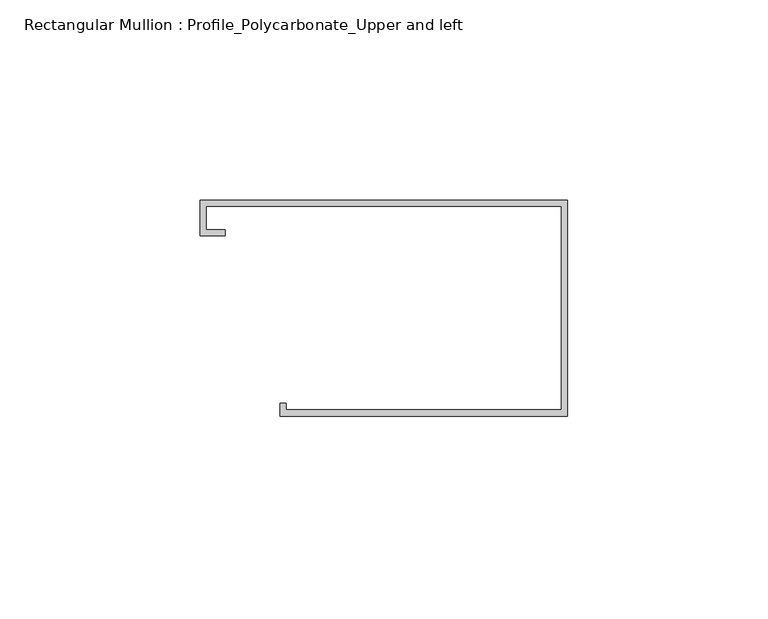
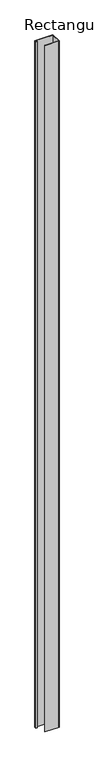
"""IFC4 building model written with IfcOpenShell, lengths in millimetres: member geometry, Rectangular Mullion : Profile_Polycarbonate_Upper and left."""

import ifcopenshell
import ifcopenshell.guid

model = None  # the IFC model being written
_history = None  # IfcOwnerHistory: only IFC2X3 demands one
_inside = {}  # id of a spatial element -> (the spatial element, [elements in it])
_under = {}  # id of a project, library or spatial element -> (it, [spatial elements below it])
_declared = {}  # id of a project -> (the project, [libraries it declares])
_typed = {}  # id of a type object -> (the type object, [elements of that type])
_made_of = {}  # id of a material, layer set ... -> (it, [elements and type objects made of it])


def new_model(schema):
    """Start an empty IFC model of exactly this schema.

    Asked for "IFC4X3", IfcOpenShell would pick the latest addendum, in which some entities
    have other attributes; the version numbers below select the first issue.
    IFC2X3 requires an IfcOwnerHistory on every rooted entity: one is made here for all.
    """
    global model, _history
    if schema == "IFC4X3":
        model = ifcopenshell.file(schema_version=(4, 3, 0, 0))
    else:
        model = ifcopenshell.file(schema=schema)
    _inside.clear()
    _under.clear()
    _declared.clear()
    _typed.clear()
    _made_of.clear()
    _history = None
    if model.schema == "IFC2X3":
        org = make("IfcOrganization", Name="unknown")
        user = make(
            "IfcPersonAndOrganization",
            ThePerson=make("IfcPerson", FamilyName="unknown"),
            TheOrganization=org,
        )
        app = make(
            "IfcApplication",
            ApplicationDeveloper=org,
            Version="unknown",
            ApplicationFullName="unknown",
            ApplicationIdentifier="unknown",
        )
        _history = make(
            "IfcOwnerHistory",
            OwningUser=user,
            OwningApplication=app,
            ChangeAction="ADDED",
            CreationDate=0,
        )
    return model


def make(cls, **values):
    """One entity of the class cls with the attributes given. An attribute that is None is left unset."""
    return model.create_entity(
        cls, **{name: value for name, value in values.items() if value is not None}
    )


def rooted(cls, **values):
    """An entity with a GlobalId (a new one), such as an element, a storey or a relation."""
    return make(cls, GlobalId=ifcopenshell.guid.new(), OwnerHistory=_history, **values)


def si_unit(unit_type, name, prefix=None):
    """IfcSIUnit, for example si_unit("LENGTHUNIT", "METRE", prefix="MILLI")."""
    return make("IfcSIUnit", UnitType=unit_type, Prefix=prefix, Name=name)


def assignment(units):
    """IfcUnitAssignment: the units of a project."""
    return None if units is None else make("IfcUnitAssignment", Units=units)


def point(xyz):
    """IfcCartesianPoint."""
    return None if xyz is None else make("IfcCartesianPoint", Coordinates=xyz)


def direction(xyz):
    """IfcDirection."""
    return None if xyz is None else make("IfcDirection", DirectionRatios=xyz)


def frame(location, z_axis=None, x_axis=None):
    """IfcAxis2Placement3D, a coordinate frame: its origin and axes. An axis left out is left unset."""
    return make(
        "IfcAxis2Placement3D",
        Location=point(location),
        Axis=direction(z_axis),
        RefDirection=direction(x_axis),
    )


def origin():
    """The frame at (0, 0, 0) with its axes left unset."""
    return frame((0.0, 0.0, 0.0))


def place(relative_to, where):
    """IfcLocalPlacement: puts the frame where relative to a parent placement (None: the world)."""
    return make(
        "IfcLocalPlacement", PlacementRelTo=relative_to, RelativePlacement=where
    )


def context(
    kind, dimensions, precision=None, world=None, true_north=None, identifier=None
):
    """IfcGeometricRepresentationContext, for example the 3D "Model" context."""
    return make(
        "IfcGeometricRepresentationContext",
        ContextIdentifier=identifier,
        ContextType=kind,
        CoordinateSpaceDimension=dimensions,
        Precision=precision,
        WorldCoordinateSystem=world,
        TrueNorth=true_north,
    )


def project(units=None, contexts=None):
    """IfcProject with its units and contexts."""
    return rooted(
        "IfcProject",
        Name="project",
        RepresentationContexts=contexts,
        UnitsInContext=assignment(units),
    )


def spatial(cls, under=None, at=None, **own):
    """A site, building, storey or space (cls), placed at a placement, below another one or the project."""
    s = rooted(cls, ObjectPlacement=at, **own)
    if under is not None:
        _under.setdefault(under.id(), (under, []))[1].append(s)
    return s


def polyline(points):
    """IfcPolyline through the points."""
    return make("IfcPolyline", Points=[point(p) for p in points])


def outline(outer, holes=None, kind="AREA"):
    """IfcArbitraryClosedProfileDef: a profile drawn as a closed curve; with holes, ...WithVoids."""
    if holes is None:
        return make("IfcArbitraryClosedProfileDef", ProfileType=kind, OuterCurve=outer)
    return make(
        "IfcArbitraryProfileDefWithVoids",
        ProfileType=kind,
        OuterCurve=outer,
        InnerCurves=holes,
    )


def extrude(swept, where, along, depth):
    """IfcExtrudedAreaSolid: the profile swept, set in the frame where, extruded along a direction by depth."""
    return make(
        "IfcExtrudedAreaSolid",
        SweptArea=swept,
        Position=where,
        ExtrudedDirection=direction(along),
        Depth=depth,
    )


def shape(context_of_items, identifier, shape_type, items):
    """IfcShapeRepresentation: the items that make up one representation, for example the "Body"."""
    return make(
        "IfcShapeRepresentation",
        ContextOfItems=context_of_items,
        RepresentationIdentifier=identifier,
        RepresentationType=shape_type,
        Items=items,
    )


def source(mapping_origin, context_of_items, identifier, shape_type, items):
    """IfcRepresentationMap: a shape defined once, which mapped items show again and again."""
    return make(
        "IfcRepresentationMap",
        MappingOrigin=mapping_origin,
        MappedRepresentation=shape(context_of_items, identifier, shape_type, items),
    )


def transform(
    local_origin,
    x_axis=None,
    y_axis=None,
    z_axis=None,
    scale=None,
    scale2=None,
    scale3=None,
    uniform=True,
):
    """IfcCartesianTransformationOperator3D, or its non-uniform kind. x_axis, y_axis, z_axis: its Axis1, 2, 3."""
    if uniform:
        return make(
            "IfcCartesianTransformationOperator3D",
            Axis1=direction(x_axis),
            Axis2=direction(y_axis),
            LocalOrigin=point(local_origin),
            Scale=scale,
            Axis3=direction(z_axis),
        )
    return make(
        "IfcCartesianTransformationOperator3DnonUniform",
        Axis1=direction(x_axis),
        Axis2=direction(y_axis),
        LocalOrigin=point(local_origin),
        Scale=scale,
        Axis3=direction(z_axis),
        Scale2=scale2,
        Scale3=scale3,
    )


def mapped(mapping_source, mapping_target):
    """IfcMappedItem: shows the shape of a source again, moved by a transform."""
    return make(
        "IfcMappedItem", MappingSource=mapping_source, MappingTarget=mapping_target
    )


def made_of(thing, what):
    """Note that an element or type object is made of a material, layer set ...; save() writes the relation."""
    if what is not None:
        _made_of.setdefault(what.id(), (what, []))[1].append(thing)
    return thing


def element(
    cls,
    number,
    at=None,
    inside=None,
    cuts=None,
    type_object=None,
    material=None,
    context=None,
    identifier="Body",
    shape_type=None,
    held_by="IfcProductDefinitionShape",
    body=None,
    shapes=None,
    **own,
):
    """One element of the class cls, such as IfcWall. Its Tag is "e" and its number.

    at: its placement. inside: the storey or other place that contains it. cuts: it is an
    opening in that element (IfcRelVoidsElement). A single representation is given by context,
    identifier, shape_type and body (its items); several are given by shapes. held_by: the class
    of the entity that holds the representations. save() writes the other relations.
    """
    e = rooted(cls, Tag="e%d" % number, ObjectPlacement=at, **own)
    if body is not None:
        shapes = [shape(context, identifier, shape_type, body)]
    if shapes is not None:
        e.Representation = make(held_by, Representations=shapes)
    if inside is not None:
        _inside.setdefault(inside.id(), (inside, []))[1].append(e)
    if cuts is not None:
        rooted(
            "IfcRelVoidsElement", RelatingBuildingElement=cuts, RelatedOpeningElement=e
        )
    if type_object is not None:
        _typed.setdefault(type_object.id(), (type_object, []))[1].append(e)
    return made_of(e, material)


def aggregate(whole, parts):
    """IfcRelAggregates: a whole, such as a stair, and the parts it consists of."""
    return rooted("IfcRelAggregates", RelatingObject=whole, RelatedObjects=parts)


def save(model, path):
    """Write the relations noted so far, then the file.

    IfcRelAggregates (storeys below a building ...), IfcRelContainedInSpatialStructure (elements
    in a storey), IfcRelDefinesByType, IfcRelAssociatesMaterial and IfcRelDeclares: one each for
    every whole, place, type object, material and project.
    """
    for whole, parts in _under.values():
        aggregate(whole, parts)
    for where, things in _inside.values():
        rooted(
            "IfcRelContainedInSpatialStructure",
            RelatedElements=things,
            RelatingStructure=where,
        )
    for kind, things in _typed.values():
        rooted("IfcRelDefinesByType", RelatedObjects=things, RelatingType=kind)
    for what, things in _made_of.values():
        rooted("IfcRelAssociatesMaterial", RelatedObjects=things, RelatingMaterial=what)
    for by, libraries in _declared.values():
        rooted("IfcRelDeclares", RelatingContext=by, RelatedDefinitions=libraries)
    model.write(path)


def rectangular_mullion_profile_polycarbonate_upper_and_left_19000c9a(model_context):
    return source(origin(), model_context, "Body", "SweptSolid", [
        extrude(outline(polyline([(0.0, 28.984575), (0.0, -25.015825), (-71.9836, -25.015825), (-71.9836, -21.840825), (-70.3961, -21.840825), (-70.3961, -23.428325), (-1.5875, -23.428325), (-1.5875, 27.397075), (-90.4113, 27.397075), (-90.4113, 21.580475), (-85.6488, 21.580475), (-85.6488, 19.992975), (-91.9988, 19.992975), (-91.9988, 28.984575), (0.0, 28.984575)])), frame((0.0, 0.0, -3695.7), z_axis=(0.0, 0.0, 1.0), x_axis=(1.0, 0.0, 0.0)), (0.0, 0.0, 1.0), 3695.7),
    ])


if __name__ == "__main__":
    model = new_model("IFC4")
    model_context = context("Model", 3, world=origin())
    ifc_project = project(units=[si_unit("LENGTHUNIT", "METRE", prefix="MILLI")], contexts=[model_context])
    site = spatial("IfcSite", under=ifc_project)
    building = spatial("IfcBuilding", under=site)
    placement = place(None, origin())
    rectangular_mullion_profile_polycarbonate_upper_and_left_shape = rectangular_mullion_profile_polycarbonate_upper_and_left_19000c9a(model_context)
    element("IfcMember", 1, ObjectType="Rectangular Mullion : Profile_Polycarbonate_Upper and left", at=placement, inside=building, context=model_context, shape_type="MappedRepresentation", body=[
        mapped(rectangular_mullion_profile_polycarbonate_upper_and_left_shape, transform((0.0, 0.0, 0.0), x_axis=(1.0, 0.0, 0.0), y_axis=(0.0, 1.0, 0.0), z_axis=(0.0, 0.0, 1.0))),
    ])
    save(model, "model.ifc")

# Revit data of these elements
# Type "Rectangular Mullion : Profile_Polycarbonate_Upper and left"
#   built-in parameter 1007322 = 0.177167 (stored number, unit not read)
#   built-in parameter 1007321 = 0.00520833 (stored number, unit not read)
#   built-in parameter 1007320 = 0 (stored number, unit not read)
